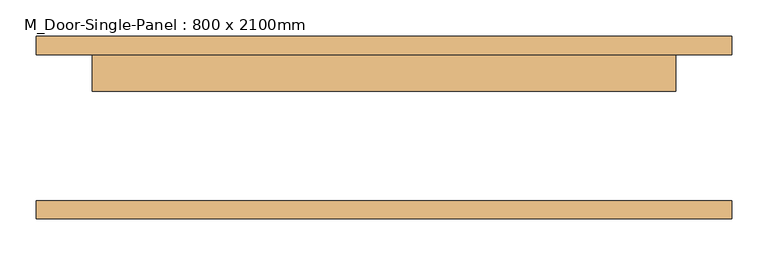
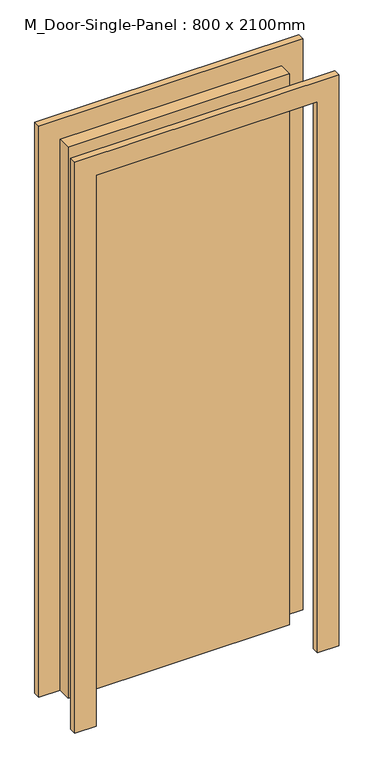
"""IFC4 building model written with IfcOpenShell, lengths in millimetres: door geometry, M_Door-Single-Panel : 800 x 2100mm."""

from ifc_helpers import new_model, si_unit, frame, origin, origin_with_axes, place, context, project, spatial, polyline, outline, extrude, source, transform, mapped, element, save


def m_door_single_panel_800_x_2100mm_e6cd55ec(model_context):
    return source(origin(), model_context, "Body", "SweptSolid", [
        extrude(outline(polyline([(400.0, 50.0), (-400.0, 50.0), (-400.0, 100.0), (400.0, 100.0), (400.0, 50.0)])), origin_with_axes(), (0.0, 0.0, 1.0), 2100.0),
        extrude(outline(polyline([(2176.2, -476.2), (0.0, -476.2), (0.0, -400.0), (2100.0, -400.0), (2100.0, 400.0), (0.0, 400.0), (0.0, 476.2), (2176.2, 476.2), (2176.2, -476.2)])), frame((0.0, 100.0, 0.0), z_axis=(0.0, 1.0, 0.0), x_axis=(0.0, 0.0, 1.0)), (0.0, 0.0, 1.0), 25.0),
        extrude(outline(polyline([(2176.2, 476.2), (2176.2, -476.2), (0.0, -476.2), (0.0, -400.0), (2100.0, -400.0), (2100.0, 400.0), (0.0, 400.0), (0.0, 476.2), (2176.2, 476.2)])), frame((0.0, -125.0, 0.0), z_axis=(0.0, 1.0, 0.0), x_axis=(0.0, 0.0, 1.0)), (0.0, 0.0, 1.0), 25.0),
    ])


if __name__ == "__main__":
    model = new_model("IFC4")
    model_context = context("Model", 3, world=origin())
    ifc_project = project(units=[si_unit("LENGTHUNIT", "METRE", prefix="MILLI")], contexts=[model_context])
    site = spatial("IfcSite", under=ifc_project)
    building = spatial("IfcBuilding", under=site)
    placement = place(None, origin())
    m_door_single_panel_800_x_2100mm_shape = m_door_single_panel_800_x_2100mm_e6cd55ec(model_context)
    element("IfcDoor", 1, ObjectType="M_Door-Single-Panel : 800 x 2100mm", at=placement, inside=building, context=model_context, shape_type="MappedRepresentation", body=[
        mapped(m_door_single_panel_800_x_2100mm_shape, transform((0.0, 0.0, 0.0), x_axis=(1.0, 0.0, 0.0), y_axis=(0.0, 1.0, 0.0), z_axis=(0.0, 0.0, 1.0))),
    ])
    save(model, "model.ifc")

# Revit data of these elements
# Type "M_Door-Single-Panel : 800 x 2100mm"
#   Type Mark = "43"
#   Construction Type Id = "DOOR"
#   Assembly Code = "C1020300"
#   Analytic Construction = "Wooden"
#   Thickness = 50 mm
#   Thermal Resistance (R) = 0.455703 (m²·K)/W
#   Swing Angle [instance default] = 90.00°
#   Heat Transfer Coefficient (U) = 2.19465 W/(m²·K)
#   Height = 2100 mm
#   Trim Projection Ext = 25 mm
#   Trim Projection Int = 25 mm
#   Trim Width = 80 mm
#   Width = 800 mm
#   Panel Material = Wood - Birch - Solid Stained Light Low Gloss
#   Trim Material = Paint - Sienna
#   Visual Light Transmittance = 0
#   Solar Heat Gain Coefficient = 0
#   Function = (empty or 0)
#   Wall Closure = (empty or 0)
# Element 1 (IfcDoor, "M_Door-Single-Panel : 800 x 2100mm")
#   Materials on its faces: "Paint - Sienna", "Wood - Birch - Solid Stained Light Low Gloss"
# Materials
#   "Wood - Birch - Solid Stained Light Low Gloss": class "Wood", colour RGB 210 159 95, transparency 0, Cost = 0
#   "Paint - Sienna": class "Miscellaneous", colour RGB 118 70 51, transparency 0, Cost = 0
